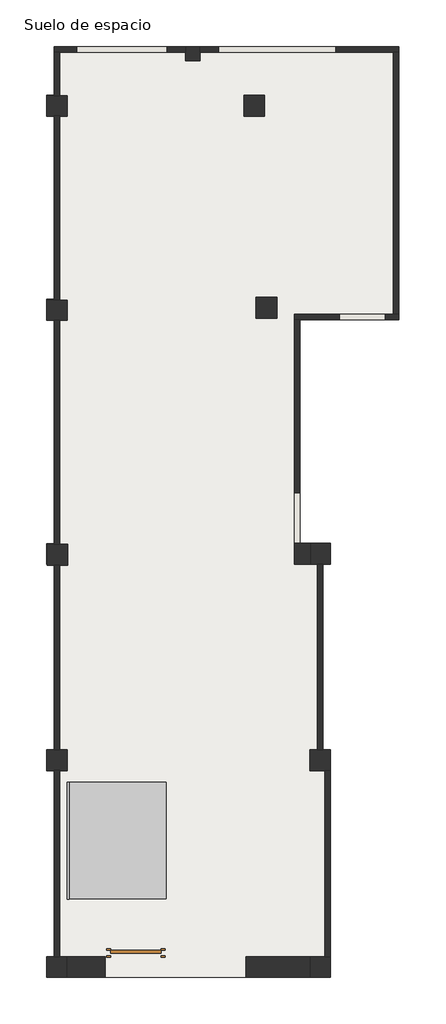
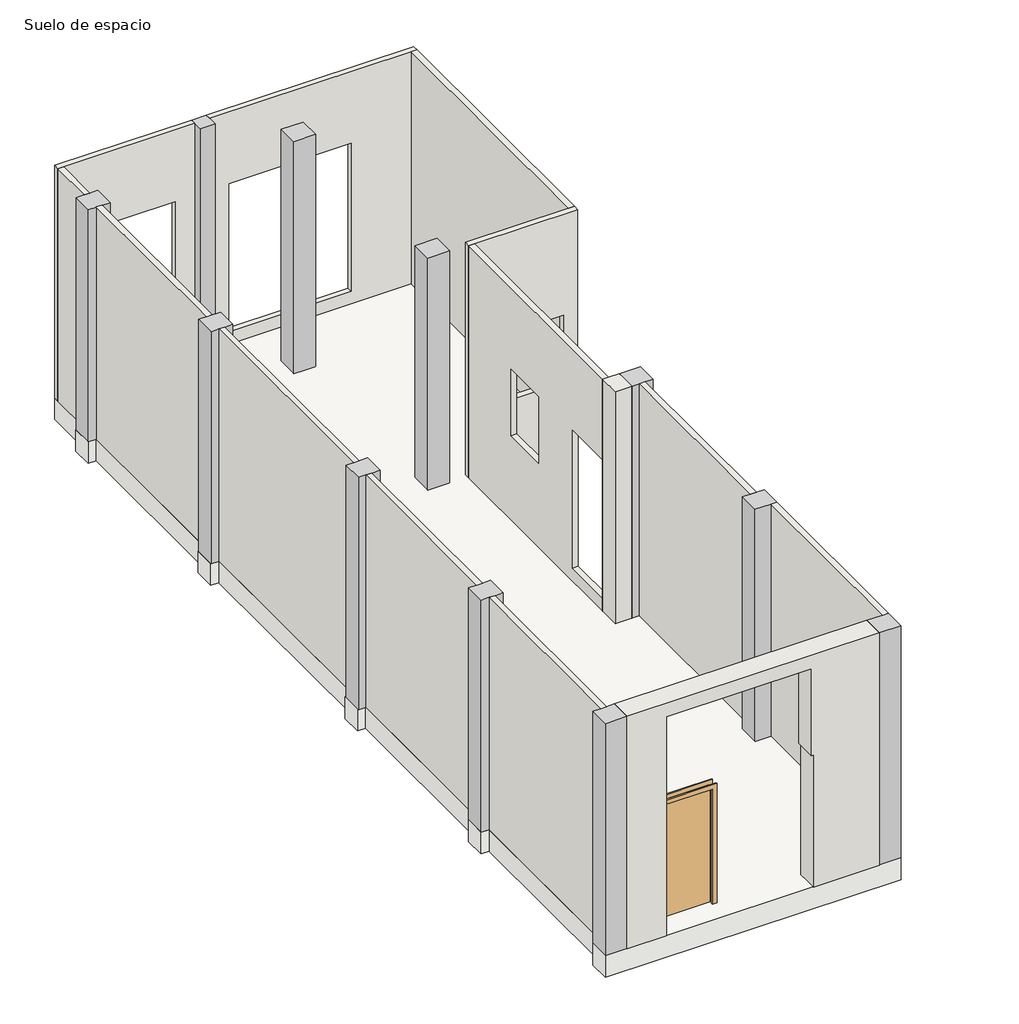
# One storey: 14 walls, 11 columns, 1 door, 1 railing, 1 ramp, 1 slab.
"""IFC4 building model written with IfcOpenShell, lengths in millimetres."""

import ifcopenshell
import ifcopenshell.guid

model = None  # the IFC model being written
_history = None  # IfcOwnerHistory: only IFC2X3 demands one
_inside = {}  # id of a spatial element -> (the spatial element, [elements in it])
_under = {}  # id of a project, library or spatial element -> (it, [spatial elements below it])
_declared = {}  # id of a project -> (the project, [libraries it declares])
_typed = {}  # id of a type object -> (the type object, [elements of that type])
_made_of = {}  # id of a material, layer set ... -> (it, [elements and type objects made of it])


def new_model(schema):
    """Start an empty IFC model of exactly this schema.

    Asked for "IFC4X3", IfcOpenShell would pick the latest addendum, in which some entities
    have other attributes; the version numbers below select the first issue.
    IFC2X3 requires an IfcOwnerHistory on every rooted entity: one is made here for all.
    """
    global model, _history
    if schema == "IFC4X3":
        model = ifcopenshell.file(schema_version=(4, 3, 0, 0))
    else:
        model = ifcopenshell.file(schema=schema)
    _inside.clear()
    _under.clear()
    _declared.clear()
    _typed.clear()
    _made_of.clear()
    _history = None
    if model.schema == "IFC2X3":
        org = make("IfcOrganization", Name="unknown")
        user = make(
            "IfcPersonAndOrganization",
            ThePerson=make("IfcPerson", FamilyName="unknown"),
            TheOrganization=org,
        )
        app = make(
            "IfcApplication",
            ApplicationDeveloper=org,
            Version="unknown",
            ApplicationFullName="unknown",
            ApplicationIdentifier="unknown",
        )
        _history = make(
            "IfcOwnerHistory",
            OwningUser=user,
            OwningApplication=app,
            ChangeAction="ADDED",
            CreationDate=0,
        )
    return model


def make(cls, **values):
    """One entity of the class cls with the attributes given. An attribute that is None is left unset."""
    return model.create_entity(
        cls, **{name: value for name, value in values.items() if value is not None}
    )


def rooted(cls, **values):
    """An entity with a GlobalId (a new one), such as an element, a storey or a relation."""
    return make(cls, GlobalId=ifcopenshell.guid.new(), OwnerHistory=_history, **values)


def si_unit(unit_type, name, prefix=None):
    """IfcSIUnit, for example si_unit("LENGTHUNIT", "METRE", prefix="MILLI")."""
    return make("IfcSIUnit", UnitType=unit_type, Prefix=prefix, Name=name)


def assignment(units):
    """IfcUnitAssignment: the units of a project."""
    return None if units is None else make("IfcUnitAssignment", Units=units)


def point(xyz):
    """IfcCartesianPoint."""
    return None if xyz is None else make("IfcCartesianPoint", Coordinates=xyz)


def direction(xyz):
    """IfcDirection."""
    return None if xyz is None else make("IfcDirection", DirectionRatios=xyz)


def frame(location, z_axis=None, x_axis=None):
    """IfcAxis2Placement3D, a coordinate frame: its origin and axes. An axis left out is left unset."""
    return make(
        "IfcAxis2Placement3D",
        Location=point(location),
        Axis=direction(z_axis),
        RefDirection=direction(x_axis),
    )


def origin():
    """The frame at (0, 0, 0) with its axes left unset."""
    return frame((0.0, 0.0, 0.0))


def origin_with_axes():
    """The frame at (0, 0, 0) with the z axis (0, 0, 1) and the x axis (1, 0, 0) written out."""
    return frame((0.0, 0.0, 0.0), z_axis=(0.0, 0.0, 1.0), x_axis=(1.0, 0.0, 0.0))


def place(relative_to, where):
    """IfcLocalPlacement: puts the frame where relative to a parent placement (None: the world)."""
    return make(
        "IfcLocalPlacement", PlacementRelTo=relative_to, RelativePlacement=where
    )


def context(
    kind, dimensions, precision=None, world=None, true_north=None, identifier=None
):
    """IfcGeometricRepresentationContext, for example the 3D "Model" context."""
    return make(
        "IfcGeometricRepresentationContext",
        ContextIdentifier=identifier,
        ContextType=kind,
        CoordinateSpaceDimension=dimensions,
        Precision=precision,
        WorldCoordinateSystem=world,
        TrueNorth=true_north,
    )


def project(units=None, contexts=None):
    """IfcProject with its units and contexts."""
    return rooted(
        "IfcProject",
        Name="project",
        RepresentationContexts=contexts,
        UnitsInContext=assignment(units),
    )


def spatial(cls, under=None, at=None, **own):
    """A site, building, storey or space (cls), placed at a placement, below another one or the project."""
    s = rooted(cls, ObjectPlacement=at, **own)
    if under is not None:
        _under.setdefault(under.id(), (under, []))[1].append(s)
    return s


def polyline(points):
    """IfcPolyline through the points."""
    return make("IfcPolyline", Points=[point(p) for p in points])


def ellipse_curve(where, semi_axis1, semi_axis2):
    """IfcEllipse in the frame where."""
    return make(
        "IfcEllipse", Position=where, SemiAxis1=semi_axis1, SemiAxis2=semi_axis2
    )


def outline(outer, holes=None, kind="AREA"):
    """IfcArbitraryClosedProfileDef: a profile drawn as a closed curve; with holes, ...WithVoids."""
    if holes is None:
        return make("IfcArbitraryClosedProfileDef", ProfileType=kind, OuterCurve=outer)
    return make(
        "IfcArbitraryProfileDefWithVoids",
        ProfileType=kind,
        OuterCurve=outer,
        InnerCurves=holes,
    )


def extrude(swept, where, along, depth):
    """IfcExtrudedAreaSolid: the profile swept, set in the frame where, extruded along a direction by depth."""
    return make(
        "IfcExtrudedAreaSolid",
        SweptArea=swept,
        Position=where,
        ExtrudedDirection=direction(along),
        Depth=depth,
    )


def faces_of(points, faces, orient=None, outer=None):
    """IfcFace entities. A face is a list of loops; a loop is a list of indices into points, from 0.

    orient and outer hold one flag for each loop. By default every Orientation is true, the
    first loop of a face is its IfcFaceOuterBound and the others are IfcFaceBound.
    """
    made = []
    for i, loops in enumerate(faces):
        bounds = []
        for j, loop in enumerate(loops):
            is_outer = j == 0 if outer is None else outer[i][j]
            bounds.append(
                make(
                    "IfcFaceOuterBound" if is_outer else "IfcFaceBound",
                    Bound=make("IfcPolyLoop", Polygon=[points[k] for k in loop]),
                    Orientation=True if orient is None else orient[i][j],
                )
            )
        made.append(make("IfcFace", Bounds=bounds))
    return made


def faceted_brep(points, faces, orient=None, outer=None, voids=None):
    """IfcFacetedBrep: a solid bounded by flat faces; with voids (closed shells), ...WithVoids."""
    shared = [point(p) for p in points]
    hull = make("IfcClosedShell", CfsFaces=faces_of(shared, faces, orient, outer))
    if voids is None:
        return make("IfcFacetedBrep", Outer=hull)
    return make(
        "IfcFacetedBrepWithVoids",
        Outer=hull,
        Voids=[
            make(cls, CfsFaces=faces_of(shared, fs, o, b)) for cls, fs, o, b in voids
        ],
    )


def shape(context_of_items, identifier, shape_type, items):
    """IfcShapeRepresentation: the items that make up one representation, for example the "Body"."""
    return make(
        "IfcShapeRepresentation",
        ContextOfItems=context_of_items,
        RepresentationIdentifier=identifier,
        RepresentationType=shape_type,
        Items=items,
    )


def source(mapping_origin, context_of_items, identifier, shape_type, items):
    """IfcRepresentationMap: a shape defined once, which mapped items show again and again."""
    return make(
        "IfcRepresentationMap",
        MappingOrigin=mapping_origin,
        MappedRepresentation=shape(context_of_items, identifier, shape_type, items),
    )


def transform(
    local_origin,
    x_axis=None,
    y_axis=None,
    z_axis=None,
    scale=None,
    scale2=None,
    scale3=None,
    uniform=True,
):
    """IfcCartesianTransformationOperator3D, or its non-uniform kind. x_axis, y_axis, z_axis: its Axis1, 2, 3."""
    if uniform:
        return make(
            "IfcCartesianTransformationOperator3D",
            Axis1=direction(x_axis),
            Axis2=direction(y_axis),
            LocalOrigin=point(local_origin),
            Scale=scale,
            Axis3=direction(z_axis),
        )
    return make(
        "IfcCartesianTransformationOperator3DnonUniform",
        Axis1=direction(x_axis),
        Axis2=direction(y_axis),
        LocalOrigin=point(local_origin),
        Scale=scale,
        Axis3=direction(z_axis),
        Scale2=scale2,
        Scale3=scale3,
    )


def mapped(mapping_source, mapping_target):
    """IfcMappedItem: shows the shape of a source again, moved by a transform."""
    return make(
        "IfcMappedItem", MappingSource=mapping_source, MappingTarget=mapping_target
    )


def made_of(thing, what):
    """Note that an element or type object is made of a material, layer set ...; save() writes the relation."""
    if what is not None:
        _made_of.setdefault(what.id(), (what, []))[1].append(thing)
    return thing


def element(
    cls,
    number,
    at=None,
    inside=None,
    cuts=None,
    type_object=None,
    material=None,
    context=None,
    identifier="Body",
    shape_type=None,
    held_by="IfcProductDefinitionShape",
    body=None,
    shapes=None,
    **own,
):
    """One element of the class cls, such as IfcWall. Its Tag is "e" and its number.

    at: its placement. inside: the storey or other place that contains it. cuts: it is an
    opening in that element (IfcRelVoidsElement). A single representation is given by context,
    identifier, shape_type and body (its items); several are given by shapes. held_by: the class
    of the entity that holds the representations. save() writes the other relations.
    """
    e = rooted(cls, Tag="e%d" % number, ObjectPlacement=at, **own)
    if body is not None:
        shapes = [shape(context, identifier, shape_type, body)]
    if shapes is not None:
        e.Representation = make(held_by, Representations=shapes)
    if inside is not None:
        _inside.setdefault(inside.id(), (inside, []))[1].append(e)
    if cuts is not None:
        rooted(
            "IfcRelVoidsElement", RelatingBuildingElement=cuts, RelatedOpeningElement=e
        )
    if type_object is not None:
        _typed.setdefault(type_object.id(), (type_object, []))[1].append(e)
    return made_of(e, material)


def aggregate(whole, parts):
    """IfcRelAggregates: a whole, such as a stair, and the parts it consists of."""
    return rooted("IfcRelAggregates", RelatingObject=whole, RelatedObjects=parts)


def save(model, path):
    """Write the relations noted so far, then the file.

    IfcRelAggregates (storeys below a building ...), IfcRelContainedInSpatialStructure (elements
    in a storey), IfcRelDefinesByType, IfcRelAssociatesMaterial and IfcRelDeclares: one each for
    every whole, place, type object, material and project.
    """
    for whole, parts in _under.values():
        aggregate(whole, parts)
    for where, things in _inside.values():
        rooted(
            "IfcRelContainedInSpatialStructure",
            RelatedElements=things,
            RelatingStructure=where,
        )
    for kind, things in _typed.values():
        rooted("IfcRelDefinesByType", RelatedObjects=things, RelatingType=kind)
    for what, things in _made_of.values():
        rooted("IfcRelAssociatesMaterial", RelatedObjects=things, RelatingMaterial=what)
    for by, libraries in _declared.values():
        rooted("IfcRelDeclares", RelatingContext=by, RelatedDefinitions=libraries)
    model.write(path)


def plane_surface(at):
    """IfcPlane: the flat surface through the origin of the frame at, square to its z axis."""
    return make("IfcPlane", Position=at)


def cylinder_surface(at, radius):
    """IfcCylindricalSurface: all points at the distance radius from the z axis of the frame at."""
    return make("IfcCylindricalSurface", Position=at, Radius=radius)


def advanced_brep(points, edges, surfaces, faces):
    """IfcAdvancedBrep: a solid bounded by faces that lie on surfaces and meet in shared edges.

    An edge is (start, end): straight between two places in points (the first is 0);
    or (start, end, curve); or (start, end, curve, False) where it runs against its curve.
    A face is (place in surfaces, loops), or (place, loops, False) where it looks against
    its surface's normal. A loop lists edges by number (the first is 1), with a minus sign
    where the edge is run from its end to its start. The first loop is the outer one.
    """
    corners = [point(p) for p in points]
    vertices = [make("IfcVertexPoint", VertexGeometry=c) for c in corners]
    made = []
    for start, end, *more in edges:
        made.append(
            make(
                "IfcEdgeCurve",
                EdgeStart=vertices[start],
                EdgeEnd=vertices[end],
                EdgeGeometry=more[0] if more else make("IfcPolyline", Points=[corners[start], corners[end]]),
                SameSense=more[1] if len(more) > 1 else True,
            )
        )
    hull = []
    for where, loops, *sense in faces:
        bounds = []
        for j, loop in enumerate(loops):
            ring = [make("IfcOrientedEdge", EdgeElement=made[abs(k) - 1], Orientation=k > 0) for k in loop]
            bounds.append(
                make(
                    "IfcFaceOuterBound" if j == 0 else "IfcFaceBound",
                    Bound=make("IfcEdgeLoop", EdgeList=ring),
                    Orientation=True,
                )
            )
        hull.append(make("IfcAdvancedFace", Bounds=bounds, FaceSurface=surfaces[where], SameSense=sense[0] if sense else True))
    return make("IfcAdvancedBrep", Outer=make("IfcClosedShell", CfsFaces=hull))


def m_rectangular_column_380_x_380mm_96b74405(model_context):
    return source(origin(), model_context, "Body", "SweptSolid", [
        extrude(outline(polyline([(190.0, 190.0), (190.0, -190.0), (-190.0, -190.0), (-190.0, 190.0), (190.0, 190.0)])), origin_with_axes(), (0.0, 0.0, 1.0), 4300.0),
    ])


def m_single_flush_0915_x_2134mm_17617764(model_context):
    return source(origin(), model_context, "Body", "SweptSolid", [
        extrude(outline(polyline([(2210.0, -533.5), (0.0, -533.5), (0.0, -457.5), (2134.0, -457.5), (2134.0, 457.5), (0.0, 457.5), (0.0, 533.5), (2210.0, 533.5), (2210.0, -533.5)])), frame((0.0, -75.0, 0.0), z_axis=(0.0, 1.0, 0.0), x_axis=(0.0, 0.0, 1.0)), (0.0, 0.0, 1.0), 25.0),
        extrude(outline(polyline([(2210.0, 533.5), (2210.0, -533.5), (0.0, -533.5), (0.0, -457.5), (2134.0, -457.5), (2134.0, 457.5), (0.0, 457.5), (0.0, 533.5), (2210.0, 533.5)])), frame((0.0, 50.0, 0.0), z_axis=(0.0, 1.0, 0.0), x_axis=(0.0, 0.0, 1.0)), (0.0, 0.0, 1.0), 25.0),
        extrude(outline(polyline([(457.5, 1.0), (457.5, -50.0), (-457.5, -50.0), (-457.5, 1.0), (457.5, 1.0)])), origin_with_axes(), (0.0, 0.0, 1.0), 2134.0),
    ])


def ramp_1_1c041b4d(model_context):
    return source(origin(), model_context, "Body", "SweptSolid", [
        extrude(outline(polyline([(-588.7354398, 0.0), (1550.939444, 178.3062403), (1550.939444, 27.7863081), (-588.7354398, -150.5199322), (-588.7354398, 0.0)])), frame((5737.3508412, 0.0, 0.0), z_axis=(1.0, 0.0, 0.0), x_axis=(0.0, 1.0, 0.0)), (0.0, 0.0, 1.0), 1790.0),
    ])


model = new_model("IFC4")

# Units and contexts
model_context = context("Model", 3, world=origin())
ifc_project = project(units=[si_unit("LENGTHUNIT", "METRE", prefix="MILLI")], contexts=[model_context])

# Site, building, storey
site = spatial("IfcSite", under=ifc_project)
building = spatial("IfcBuilding", under=site)
storey = spatial("IfcBuildingStorey", under=building, Name="Suelo de espacio", Elevation=0.0)

# Columns
placement = place(None, origin())
element("IfcColumn", 1, ObjectType="M_Rectangular Column : 260 x 260mm", at=placement, inside=storey, context=model_context, shape_type="Brep", body=[
    faceted_brep([(8142.3508412, 14950.939444, 4300.0), (7882.3508412, 14950.939444, 4300.0), (7882.3508412, 14850.939444, 4300.0), (7882.3508412, 14690.939444, 4300.0), (8142.3508412, 14690.939444, 4300.0), (8142.3508412, 14850.939444, 4300.0), (8142.3508412, 14950.939444, 0.0), (8142.3508412, 14850.939444, 0.0), (8142.3508412, 14690.939444, 0.0), (7882.3508412, 14690.939444, 0.0), (7882.3508412, 14850.939444, 0.0), (7882.3508412, 14950.939444, 0.0)], [[[0, 1, 2, 3, 4, 5]], [[6, 7, 8, 9, 10, 11]], [[1, 0, 6, 11]], [[3, 2, 1, 11, 10, 9]], [[4, 3, 9, 8]], [[0, 5, 4, 8, 7, 6]]]),
])
element("IfcColumn", 2, ObjectType="M_Rectangular Column : 380 x 370mm", at=placement, inside=storey, context=model_context, shape_type="Brep", body=[
    faceted_brep([(5722.3508412, 10330.939444, 4300.0), (5342.3508412, 10330.939444, 4300.0), (5342.3508412, 9960.939444, 4300.0), (5482.3508412, 9960.939444, 4300.0), (5582.3508412, 9960.939444, 4300.0), (5722.3508412, 9960.939444, 4300.0), (5722.3508412, 10330.939444, 0.0), (5722.3508412, 9960.939444, 0.0), (5582.3508412, 9960.939444, 0.0), (5482.3508412, 9960.939444, 0.0), (5342.3508412, 9960.939444, 0.0), (5342.3508412, 10330.939444, 0.0)], [[[0, 1, 2, 3, 4, 5]], [[6, 7, 8, 9, 10, 11]], [[1, 0, 6, 11]], [[2, 1, 11, 10]], [[5, 4, 3, 2, 10, 9, 8, 7]], [[0, 5, 7, 6]]]),
])
element("IfcColumn", 3, ObjectType="M_Rectangular Column : 380 x 370mm", at=placement, inside=storey, context=model_context, shape_type="Brep", body=[
    faceted_brep([(5722.3508412, 14050.939444, 4300.0), (5582.3508412, 14050.939444, 4300.0), (5482.3508412, 14050.939444, 4300.0), (5342.3508412, 14050.939444, 4300.0), (5342.3508412, 13680.939444, 4300.0), (5482.3508412, 13680.939444, 4300.0), (5482.3508412, 13685.939444, 4300.0), (5582.3508412, 13685.939444, 4300.0), (5582.3508412, 13680.939444, 4300.0), (5722.3508412, 13680.939444, 4300.0), (5722.3508412, 14050.939444, 0.0), (5722.3508412, 13680.939444, 0.0), (5582.3508412, 13680.939444, 0.0), (5582.3508412, 13685.939444, 0.0), (5482.3508412, 13685.939444, 0.0), (5482.3508412, 13680.939444, 0.0), (5342.3508412, 13680.939444, 0.0), (5342.3508412, 14050.939444, 0.0), (5482.3508412, 14050.939444, 0.0), (5582.3508412, 14050.939444, 0.0)], [[[0, 1, 2, 3, 4, 5, 6, 7, 8, 9]], [[10, 11, 12, 13, 14, 15, 16, 17, 18, 19]], [[3, 2, 1, 0, 10, 19, 18, 17]], [[4, 3, 17, 16]], [[4, 16, 15, 5]], [[0, 9, 11, 10]], [[7, 13, 12, 8]], [[14, 6, 5, 15]], [[13, 7, 6, 14]], [[11, 9, 8, 12]]]),
])
element("IfcColumn", 4, ObjectType="M_Rectangular Column : 380 x 380mm", at=placement, inside=storey, context=model_context, shape_type="Brep", body=[
    faceted_brep([(5722.3508412, -1629.060556, 4300.0), (5582.3508412, -1629.060556, 4300.0), (5482.3508412, -1629.060556, 4300.0), (5342.3508412, -1629.060556, 4300.0), (5342.3508412, -2009.060556, 4300.0), (5722.3508412, -2009.060556, 4300.0), (5722.3508412, -1629.060556, 0.0), (5722.3508412, -2009.060556, 0.0), (5342.3508412, -2009.060556, 0.0), (5342.3508412, -1629.060556, 0.0), (5482.3508412, -1629.060556, 0.0), (5582.3508412, -1629.060556, 0.0)], [[[0, 1, 2, 3, 4, 5]], [[6, 7, 8, 9, 10, 11]], [[3, 2, 1, 0, 6, 11, 10, 9]], [[4, 3, 9, 8]], [[5, 4, 8, 7]], [[0, 5, 7, 6]]]),
])
element("IfcColumn", 5, ObjectType="M_Rectangular Column : 380 x 380mm", at=placement, inside=storey, context=model_context, shape_type="Brep", body=[
    faceted_brep([(10522.3508412, -1629.060556, 4300.0), (10422.3508412, -1629.060556, 4300.0), (10142.3508412, -1629.060556, 4300.0), (10142.3508412, -2009.060556, 4300.0), (10522.3508412, -2009.060556, 4300.0), (10522.3508412, -1629.060556, 0.0), (10522.3508412, -2009.060556, 0.0), (10142.3508412, -2009.060556, 0.0), (10142.3508412, -1629.060556, 0.0), (10422.3508412, -1629.060556, 0.0)], [[[0, 1, 2, 3, 4]], [[5, 6, 7, 8, 9]], [[2, 1, 0, 5, 9, 8]], [[3, 2, 8, 7]], [[4, 3, 7, 6]], [[0, 4, 6, 5]]]),
])
element("IfcColumn", 6, ObjectType="M_Rectangular Column : 380 x 380mm", at=placement, inside=storey, context=model_context, shape_type="Brep", body=[
    faceted_brep([(5722.3508412, 2140.939444, 4300.0), (5582.3508412, 2140.939444, 4300.0), (5482.3508412, 2140.939444, 4300.0), (5342.3508412, 2140.939444, 4300.0), (5342.3508412, 1760.939444, 4300.0), (5482.3508412, 1760.939444, 4300.0), (5482.3508412, 1761.3849652, 4300.0), (5582.3508412, 1761.3849652, 4300.0), (5582.3508412, 1760.939444, 4300.0), (5722.3508412, 1760.939444, 4300.0), (5722.3508412, 2140.939444, 0.0), (5722.3508412, 1760.939444, 0.0), (5582.3508412, 1760.939444, 0.0), (5582.3508412, 1761.3849652, 0.0), (5482.3508412, 1761.3849652, 0.0), (5482.3508412, 1760.939444, 0.0), (5342.3508412, 1760.939444, 0.0), (5342.3508412, 2140.939444, 0.0), (5482.3508412, 2140.939444, 0.0), (5582.3508412, 2140.939444, 0.0)], [[[0, 1, 2, 3, 4, 5, 6, 7, 8, 9]], [[10, 11, 12, 13, 14, 15, 16, 17, 18, 19]], [[3, 2, 1, 0, 10, 19, 18, 17]], [[4, 3, 17, 16]], [[4, 16, 15, 5]], [[0, 9, 11, 10]], [[7, 13, 12, 8]], [[14, 6, 5, 15]], [[11, 9, 8, 12]], [[13, 7, 6, 14]]]),
])
element("IfcColumn", 7, ObjectType="M_Rectangular Column : 380 x 380mm", at=placement, inside=storey, context=model_context, shape_type="Brep", body=[
    faceted_brep([(10522.3508412, 2140.939444, 4300.0), (10382.3508412, 2140.939444, 4300.0), (10282.3508412, 2140.939444, 4300.0), (10142.3508412, 2140.939444, 4300.0), (10142.3508412, 1760.939444, 4300.0), (10422.3508412, 1760.939444, 4300.0), (10522.3508412, 1760.939444, 4300.0), (10522.3508412, 2140.939444, 0.0), (10522.3508412, 1760.939444, 0.0), (10422.3508412, 1760.939444, 0.0), (10142.3508412, 1760.939444, 0.0), (10142.3508412, 2140.939444, 0.0), (10282.3508412, 2140.939444, 0.0), (10382.3508412, 2140.939444, 0.0)], [[[0, 1, 2, 3, 4, 5, 6]], [[7, 8, 9, 10, 11, 12, 13]], [[3, 2, 1, 0, 7, 13, 12, 11]], [[4, 3, 11, 10]], [[6, 5, 4, 10, 9, 8]], [[0, 6, 8, 7]]]),
])
element("IfcColumn", 8, ObjectType="M_Rectangular Column : 380 x 380mm", at=placement, inside=storey, context=model_context, shape_type="Brep", body=[
    faceted_brep([(5732.3508412, 5880.939444, 4300.0), (5582.3508412, 5880.939444, 4300.0), (5482.3508412, 5880.939444, 4300.0), (5352.3508412, 5880.939444, 4300.0), (5352.3508412, 5500.939444, 4300.0), (5482.3508412, 5500.939444, 4300.0), (5582.3508412, 5500.939444, 4300.0), (5732.3508412, 5500.939444, 4300.0), (5732.3508412, 5880.939444, 0.0), (5732.3508412, 5500.939444, 0.0), (5582.3508412, 5500.939444, 0.0), (5482.3508412, 5500.939444, 0.0), (5352.3508412, 5500.939444, 0.0), (5352.3508412, 5880.939444, 0.0), (5482.3508412, 5880.939444, 0.0), (5582.3508412, 5880.939444, 0.0)], [[[0, 1, 2, 3, 4, 5, 6, 7]], [[8, 9, 10, 11, 12, 13, 14, 15]], [[3, 2, 1, 0, 8, 15, 14, 13]], [[4, 3, 13, 12]], [[7, 6, 5, 4, 12, 11, 10, 9]], [[0, 7, 9, 8]]]),
])
element("IfcColumn", 9, ObjectType="M_Rectangular Column : 380 x 380mm", at=placement, inside=storey, context=model_context, shape_type="Brep", body=[
    faceted_brep([(10522.3508412, 5520.939444, 4300.0), (10522.3508412, 5900.939444, 4300.0), (10152.3508412, 5900.939444, 4300.0), (10152.3508412, 5520.939444, 4300.0), (10282.3508412, 5520.939444, 4300.0), (10382.3508412, 5520.939444, 4300.0), (10522.3508412, 5900.939444, 0.0), (10522.3508412, 5520.939444, 0.0), (10382.3508412, 5520.939444, 0.0), (10282.3508412, 5520.939444, 0.0), (10152.3508412, 5520.939444, 0.0), (10152.3508412, 5900.939444, 0.0)], [[[0, 1, 2, 3, 4, 5]], [[6, 7, 8, 9, 10, 11]], [[1, 6, 11, 2]], [[7, 0, 5, 4, 3, 10, 9, 8]], [[1, 0, 7, 6]], [[3, 2, 11, 10]]]),
])
m_rectangular_column_380_x_380mm_shape = m_rectangular_column_380_x_380mm_96b74405(model_context)
element("IfcColumn", 10, ObjectType="M_Rectangular Column : 380 x 380mm", at=placement, inside=storey, context=model_context, shape_type="MappedRepresentation", body=[
    mapped(m_rectangular_column_380_x_380mm_shape, transform((9132.3508412, 13870.939444, 0.0), x_axis=(1.0, 0.0, 0.0), y_axis=(0.0, 1.0, 0.0), z_axis=(0.0, 0.0, 1.0))),
])
element("IfcColumn", 11, ObjectType="M_Rectangular Column : 380 x 380mm", at=placement, inside=storey, context=model_context, shape_type="MappedRepresentation", body=[
    mapped(m_rectangular_column_380_x_380mm_shape, transform((9352.3508412, 10190.939444, 0.0), x_axis=(1.0, 0.0, 0.0), y_axis=(0.0, 1.0, 0.0), z_axis=(0.0, 0.0, 1.0))),
])

# Door
m_single_flush_0915_x_2134mm_shape = m_single_flush_0915_x_2134mm_17617764(model_context)
element("IfcDoor", 12, ObjectType="M_Single-Flush : 0915 x 2134mm", at=placement, inside=storey, context=model_context, shape_type="MappedRepresentation", body=[
    mapped(m_single_flush_0915_x_2134mm_shape, transform((6972.3508412, -1564.060556, 0.0), x_axis=(-1.0, 0.0, 0.0), y_axis=(0.0, -1.0, 0.0), z_axis=(0.0, 0.0, 1.0))),
])

# Railing
element("IfcRailing", 13, ObjectType="900mm Pipe", at=placement, inside=storey, context=model_context, shape_type="AdvancedBrep", body=[
    advanced_brep(
    [(5757.3508412, -588.7354398, 879.9306757), (5717.3508412, -588.7354398, 879.9306757), (5757.3508412, 1550.939444, 1058.236916), (5717.3508412, 1550.939444, 1058.236916)],
    [
        (0, 1, ellipse_curve(frame((5737.3508412, -588.7354398, 879.9306757), z_axis=(0.0, -1.0, 0.0), x_axis=(0.0, 0.0, -0.9999999999999999)), 20.0693243, 20.0)),
        (1, 0, ellipse_curve(frame((5737.3508412, -588.7354398, 879.9306757), z_axis=(0.0, -1.0, 0.0), x_axis=(0.0, 0.0, -0.9999999999999999)), 20.0693243, 20.0)),
        (2, 3, ellipse_curve(frame((5737.3508412, 1550.939444, 1058.236916), z_axis=(0.0, 1.0, 0.0), x_axis=(0.0, 0.0, -0.9999999999999999)), 20.0693243, 20.0)),
        (3, 2, ellipse_curve(frame((5737.3508412, 1550.939444, 1058.236916), z_axis=(0.0, 1.0, 0.0), x_axis=(0.0, 0.0, -0.9999999999999999)), 20.0693243, 20.0)),
        (0, 2),
        (3, 1),
    ],
    [
        plane_surface(frame((5737.3508412, -588.7354398, 900.0), z_axis=(0.0, -1.0, 0.0), x_axis=(0.0, 0.0, 1.0))),
        plane_surface(frame((5737.3508412, 1550.939444, 1078.3062403), z_axis=(0.0, 1.0, 0.0), x_axis=(0.0, 0.0, 1.0))),
        cylinder_surface(frame((5737.3508412, -587.0745302, 880.0690848), z_axis=(0.0, -0.9965457582448797, -0.08304547985373997), x_axis=(-1.0, 0.0, 0.0)), 20.0),
    ],
    [
        (0, [[1, 2]]),
        (1, [[3, 4]]),
        (2, [[-1, 5, -4, 6]]),
        (2, [[-2, -6, -3, -5]]),
    ],
),
    advanced_brep(
    [(5722.3508412, -588.7354398, 759.9480068), (5752.3508412, -588.7354398, 759.9480068), (5722.3508412, 1550.939444, 938.2542471), (5752.3508412, 1550.939444, 938.2542471)],
    [
        (0, 1, ellipse_curve(frame((5737.3508412, -588.7354398, 759.9480068), z_axis=(0.0, -1.0, 0.0), x_axis=(0.0, 0.0, -1.0)), 15.0519932, 15.0)),
        (1, 0, ellipse_curve(frame((5737.3508412, -588.7354398, 759.9480068), z_axis=(0.0, -1.0, 0.0), x_axis=(0.0, 0.0, -1.0)), 15.0519932, 15.0)),
        (2, 3, ellipse_curve(frame((5737.3508412, 1550.939444, 938.2542471), z_axis=(0.0, 1.0, 0.0), x_axis=(0.0, 0.0, -1.0)), 15.0519932, 15.0)),
        (3, 2, ellipse_curve(frame((5737.3508412, 1550.939444, 938.2542471), z_axis=(0.0, 1.0, 0.0), x_axis=(0.0, 0.0, -1.0)), 15.0519932, 15.0)),
        (0, 2),
        (3, 1),
    ],
    [
        plane_surface(frame((5737.3508412, -588.7354398, 775.0), z_axis=(0.0, -1.0, 0.0), x_axis=(0.0, 0.0, 1.0))),
        plane_surface(frame((5737.3508412, 1550.939444, 953.3062403), z_axis=(0.0, 1.0, 0.0), x_axis=(0.0, 0.0, 1.0))),
        cylinder_surface(frame((5737.3508412, -587.4897576, 760.0518136), z_axis=(0.0, -0.9965457582448797, -0.08304547985373999), x_axis=(1.0, 0.0, 0.0)), 15.0),
    ],
    [
        (0, [[1, 2]]),
        (1, [[3, 4]]),
        (2, [[-1, 5, -4, 6]]),
        (2, [[-2, -6, -3, -5]]),
    ],
),
    advanced_brep(
    [(5722.3508412, -588.7354398, 634.9480068), (5752.3508412, -588.7354398, 634.9480068), (5722.3508412, 1550.939444, 813.2542471), (5752.3508412, 1550.939444, 813.2542471)],
    [
        (0, 1, ellipse_curve(frame((5737.3508412, -588.7354398, 634.9480068), z_axis=(0.0, -1.0, 0.0), x_axis=(0.0, 0.0, -1.0)), 15.0519932, 15.0)),
        (1, 0, ellipse_curve(frame((5737.3508412, -588.7354398, 634.9480068), z_axis=(0.0, -1.0, 0.0), x_axis=(0.0, 0.0, -1.0)), 15.0519932, 15.0)),
        (2, 3, ellipse_curve(frame((5737.3508412, 1550.939444, 813.2542471), z_axis=(0.0, 1.0, 0.0), x_axis=(0.0, 0.0, -1.0)), 15.0519932, 15.0)),
        (3, 2, ellipse_curve(frame((5737.3508412, 1550.939444, 813.2542471), z_axis=(0.0, 1.0, 0.0), x_axis=(0.0, 0.0, -1.0)), 15.0519932, 15.0)),
        (0, 2),
        (3, 1),
    ],
    [
        plane_surface(frame((5737.3508412, -588.7354398, 650.0), z_axis=(0.0, -1.0, 0.0), x_axis=(0.0, 0.0, 1.0))),
        plane_surface(frame((5737.3508412, 1550.939444, 828.3062403), z_axis=(0.0, 1.0, 0.0), x_axis=(0.0, 0.0, 1.0))),
        cylinder_surface(frame((5737.3508412, -587.4897576, 635.0518136), z_axis=(0.0, -0.9965457582448797, -0.08304547985373999), x_axis=(1.0, 0.0, 0.0)), 15.0),
    ],
    [
        (0, [[1, 2]]),
        (1, [[3, 4]]),
        (2, [[-1, 5, -4, 6]]),
        (2, [[-2, -6, -3, -5]]),
    ],
),
    advanced_brep(
    [(5722.3508412, -588.7354398, 509.9480068), (5752.3508412, -588.7354398, 509.9480068), (5722.3508412, 1550.939444, 688.2542471), (5752.3508412, 1550.939444, 688.2542471)],
    [
        (0, 1, ellipse_curve(frame((5737.3508412, -588.7354398, 509.9480068), z_axis=(0.0, -1.0, 0.0), x_axis=(0.0, 0.0, -1.0)), 15.0519932, 15.0)),
        (1, 0, ellipse_curve(frame((5737.3508412, -588.7354398, 509.9480068), z_axis=(0.0, -1.0, 0.0), x_axis=(0.0, 0.0, -1.0)), 15.0519932, 15.0)),
        (2, 3, ellipse_curve(frame((5737.3508412, 1550.939444, 688.2542471), z_axis=(0.0, 1.0, 0.0), x_axis=(0.0, 0.0, -1.0)), 15.0519932, 15.0)),
        (3, 2, ellipse_curve(frame((5737.3508412, 1550.939444, 688.2542471), z_axis=(0.0, 1.0, 0.0), x_axis=(0.0, 0.0, -1.0)), 15.0519932, 15.0)),
        (0, 2),
        (3, 1),
    ],
    [
        plane_surface(frame((5737.3508412, -588.7354398, 525.0), z_axis=(0.0, -1.0, 0.0), x_axis=(0.0, 0.0, 1.0))),
        plane_surface(frame((5737.3508412, 1550.939444, 703.3062403), z_axis=(0.0, 1.0, 0.0), x_axis=(0.0, 0.0, 1.0))),
        cylinder_surface(frame((5737.3508412, -587.4897576, 510.0518136), z_axis=(0.0, -0.9965457582448797, -0.08304547985373999), x_axis=(1.0, 0.0, 0.0)), 15.0),
    ],
    [
        (0, [[1, 2]]),
        (1, [[3, 4]]),
        (2, [[-1, 5, -4, 6]]),
        (2, [[-2, -6, -3, -5]]),
    ],
),
    advanced_brep(
    [(5722.3508412, -588.7354398, 384.9480068), (5752.3508412, -588.7354398, 384.9480068), (5722.3508412, 1550.939444, 563.2542471), (5752.3508412, 1550.939444, 563.2542471)],
    [
        (0, 1, ellipse_curve(frame((5737.3508412, -588.7354398, 384.9480068), z_axis=(0.0, -1.0, 0.0), x_axis=(0.0, 0.0, -1.0)), 15.0519932, 15.0)),
        (1, 0, ellipse_curve(frame((5737.3508412, -588.7354398, 384.9480068), z_axis=(0.0, -1.0, 0.0), x_axis=(0.0, 0.0, -1.0)), 15.0519932, 15.0)),
        (2, 3, ellipse_curve(frame((5737.3508412, 1550.939444, 563.2542471), z_axis=(0.0, 1.0, 0.0), x_axis=(0.0, 0.0, -1.0)), 15.0519932, 15.0)),
        (3, 2, ellipse_curve(frame((5737.3508412, 1550.939444, 563.2542471), z_axis=(0.0, 1.0, 0.0), x_axis=(0.0, 0.0, -1.0)), 15.0519932, 15.0)),
        (0, 2),
        (3, 1),
    ],
    [
        plane_surface(frame((5737.3508412, -588.7354398, 400.0), z_axis=(0.0, -1.0, 0.0), x_axis=(0.0, 0.0, 1.0))),
        plane_surface(frame((5737.3508412, 1550.939444, 578.3062403), z_axis=(0.0, 1.0, 0.0), x_axis=(0.0, 0.0, 1.0))),
        cylinder_surface(frame((5737.3508412, -587.4897576, 385.0518136), z_axis=(0.0, -0.9965457582448797, -0.08304547985373996), x_axis=(1.0, 0.0, 0.0)), 15.0),
    ],
    [
        (0, [[1, 2]]),
        (1, [[3, 4]]),
        (2, [[-1, 5, -4, 6]]),
        (2, [[-2, -6, -3, -5]]),
    ],
),
    advanced_brep(
    [(5722.3508412, -588.7354398, 259.9480068), (5752.3508412, -588.7354398, 259.9480068), (5722.3508412, 1550.939444, 438.2542471), (5752.3508412, 1550.939444, 438.2542471)],
    [
        (0, 1, ellipse_curve(frame((5737.3508412, -588.7354398, 259.9480068), z_axis=(0.0, -1.0, 0.0), x_axis=(0.0, 0.0, -1.0)), 15.0519932, 15.0)),
        (1, 0, ellipse_curve(frame((5737.3508412, -588.7354398, 259.9480068), z_axis=(0.0, -1.0, 0.0), x_axis=(0.0, 0.0, -1.0)), 15.0519932, 15.0)),
        (2, 3, ellipse_curve(frame((5737.3508412, 1550.939444, 438.2542471), z_axis=(0.0, 1.0, 0.0), x_axis=(0.0, 0.0, -1.0)), 15.0519932, 15.0)),
        (3, 2, ellipse_curve(frame((5737.3508412, 1550.939444, 438.2542471), z_axis=(0.0, 1.0, 0.0), x_axis=(0.0, 0.0, -1.0)), 15.0519932, 15.0)),
        (0, 2),
        (3, 1),
    ],
    [
        plane_surface(frame((5737.3508412, -588.7354398, 275.0), z_axis=(0.0, -1.0, 0.0), x_axis=(0.0, 0.0, 1.0))),
        plane_surface(frame((5737.3508412, 1550.939444, 453.3062403), z_axis=(0.0, 1.0, 0.0), x_axis=(0.0, 0.0, 1.0))),
        cylinder_surface(frame((5737.3508412, -587.4897576, 260.0518136), z_axis=(0.0, -0.9965457582448797, -0.08304547985373996), x_axis=(1.0, 0.0, 0.0)), 15.0),
    ],
    [
        (0, [[1, 2]]),
        (1, [[3, 4]]),
        (2, [[-1, 5, -4, 6]]),
        (2, [[-2, -6, -3, -5]]),
    ],
),
    advanced_brep(
    [(5722.3508412, -588.7354398, 134.9480068), (5752.3508412, -588.7354398, 134.9480068), (5722.3508412, 1550.939444, 313.2542471), (5752.3508412, 1550.939444, 313.2542471)],
    [
        (0, 1, ellipse_curve(frame((5737.3508412, -588.7354398, 134.9480068), z_axis=(0.0, -1.0, 0.0), x_axis=(0.0, 0.0, -1.0)), 15.0519932, 15.0)),
        (1, 0, ellipse_curve(frame((5737.3508412, -588.7354398, 134.9480068), z_axis=(0.0, -1.0, 0.0), x_axis=(0.0, 0.0, -1.0)), 15.0519932, 15.0)),
        (2, 3, ellipse_curve(frame((5737.3508412, 1550.939444, 313.2542471), z_axis=(0.0, 1.0, 0.0), x_axis=(0.0, 0.0, -1.0)), 15.0519932, 15.0)),
        (3, 2, ellipse_curve(frame((5737.3508412, 1550.939444, 313.2542471), z_axis=(0.0, 1.0, 0.0), x_axis=(0.0, 0.0, -1.0)), 15.0519932, 15.0)),
        (0, 2),
        (3, 1),
    ],
    [
        plane_surface(frame((5737.3508412, -588.7354398, 150.0), z_axis=(0.0, -1.0, 0.0), x_axis=(0.0, 0.0, 1.0))),
        plane_surface(frame((5737.3508412, 1550.939444, 328.3062403), z_axis=(0.0, 1.0, 0.0), x_axis=(0.0, 0.0, 1.0))),
        cylinder_surface(frame((5737.3508412, -587.4897576, 135.0518136), z_axis=(0.0, -0.9965457582448797, -0.08304547985373996), x_axis=(1.0, 0.0, 0.0)), 15.0),
    ],
    [
        (0, [[1, 2]]),
        (1, [[3, 4]]),
        (2, [[-1, 5, -4, 6]]),
        (2, [[-2, -6, -3, -5]]),
    ],
),
    advanced_brep(
    [(5749.8508412, 1411.2645602, 1026.5280181), (5749.8508412, 1411.2645602, 166.6666667), (5724.8508412, 1411.2645602, 166.6666667), (5724.8508412, 1411.2645602, 1026.5280181)],
    [
        (0, 1),
        (1, 2, ellipse_curve(frame((5737.3508412, 1411.2645602, 166.6666667), z_axis=(0.0, -0.08304547985373995, 0.9965457582448797), x_axis=(0.0, 0.9965457582448798, 0.08304547985373882)), 12.5433277, 12.5)),
        (2, 3),
        (3, 0, ellipse_curve(frame((5737.3508412, 1411.2645602, 1026.5280181), z_axis=(0.0, 0.08304547985373997, -0.9965457582448797), x_axis=(0.0, 0.9965457582448797, 0.0830454798537388)), 12.5433277, 12.5)),
        (0, 3, ellipse_curve(frame((5737.3508412, 1411.2645602, 1026.5280181), z_axis=(0.0, 0.08304547985373997, -0.9965457582448797), x_axis=(0.0, 0.9965457582448797, 0.0830454798537388)), 12.5433277, 12.5)),
        (2, 1, ellipse_curve(frame((5737.3508412, 1411.2645602, 166.6666667), z_axis=(0.0, -0.08304547985373995, 0.9965457582448797), x_axis=(0.0, 0.9965457582448798, 0.08304547985373882)), 12.5433277, 12.5)),
    ],
    [
        cylinder_surface(frame((5737.3508412, 1411.2645602, 66.6666667), z_axis=(0.0, 0.0, 1.0), x_axis=(-1.0, 0.0, 0.0)), 12.5),
        plane_surface(frame((5712.3508412, 1436.2645602, 1028.6113514), z_axis=(0.0, -0.08304547985373997, 0.9965457582448797), x_axis=(1.0, 0.0, 0.0))),
        plane_surface(frame((5712.3508412, 1386.2645602, 164.5833333), z_axis=(0.0, 0.08304547985373995, -0.9965457582448797), x_axis=(1.0, 0.0, 0.0))),
    ],
    [
        (0, [[1, 2, 3, 4]]),
        (0, [[-1, 5, -3, 6]]),
        (1, [[-4, -5]]),
        (2, [[-2, -6]]),
    ],
),
    advanced_brep(
    [(5749.8508412, 411.2645602, 943.1946847), (5749.8508412, 411.2645602, 83.3333333), (5724.8508412, 411.2645602, 83.3333333), (5724.8508412, 411.2645602, 943.1946847)],
    [
        (0, 1),
        (1, 2, ellipse_curve(frame((5737.3508412, 411.2645602, 83.3333333), z_axis=(0.0, -0.08304547985373995, 0.9965457582448797), x_axis=(0.0, 0.9965457582448798, 0.08304547985373882)), 12.5433277, 12.5)),
        (2, 3),
        (3, 0, ellipse_curve(frame((5737.3508412, 411.2645602, 943.1946847), z_axis=(0.0, 0.08304547985373997, -0.9965457582448797), x_axis=(0.0, 0.9965457582448797, 0.0830454798537388)), 12.5433277, 12.5)),
        (0, 3, ellipse_curve(frame((5737.3508412, 411.2645602, 943.1946847), z_axis=(0.0, 0.08304547985373997, -0.9965457582448797), x_axis=(0.0, 0.9965457582448797, 0.0830454798537388)), 12.5433277, 12.5)),
        (2, 1, ellipse_curve(frame((5737.3508412, 411.2645602, 83.3333333), z_axis=(0.0, -0.08304547985373995, 0.9965457582448797), x_axis=(0.0, 0.9965457582448798, 0.08304547985373882)), 12.5433277, 12.5)),
    ],
    [
        cylinder_surface(frame((5737.3508412, 411.2645602, -16.6666667), z_axis=(0.0, 0.0, 1.0), x_axis=(-1.0, 0.0, 0.0)), 12.5),
        plane_surface(frame((5712.3508412, 436.2645602, 945.2780181), z_axis=(0.0, -0.08304547985373997, 0.9965457582448797), x_axis=(1.0, 0.0, 0.0))),
        plane_surface(frame((5712.3508412, 386.2645602, 81.25), z_axis=(0.0, 0.08304547985373995, -0.9965457582448797), x_axis=(1.0, 0.0, 0.0))),
    ],
    [
        (0, [[1, 2, 3, 4]]),
        (0, [[-1, 5, -3, 6]]),
        (1, [[-4, -5]]),
        (2, [[-2, -6]]),
    ],
),
    advanced_brep(
    [(5749.8508412, 1538.439444, 1037.1259251), (5749.8508412, 1538.439444, 177.2645736), (5724.8508412, 1538.439444, 177.2645736), (5724.8508412, 1538.439444, 1037.1259251)],
    [
        (0, 1),
        (1, 2, ellipse_curve(frame((5737.3508412, 1538.439444, 177.2645736), z_axis=(0.0, -0.08304547985373995, 0.9965457582448797), x_axis=(0.0, 0.9965457582448798, 0.08304547985373882)), 12.5433277, 12.5)),
        (2, 3),
        (3, 0, ellipse_curve(frame((5737.3508412, 1538.439444, 1037.1259251), z_axis=(0.0, 0.08304547985373997, -0.9965457582448797), x_axis=(0.0, 0.9965457582448797, 0.0830454798537388)), 12.5433277, 12.5)),
        (0, 3, ellipse_curve(frame((5737.3508412, 1538.439444, 1037.1259251), z_axis=(0.0, 0.08304547985373997, -0.9965457582448797), x_axis=(0.0, 0.9965457582448797, 0.0830454798537388)), 12.5433277, 12.5)),
        (2, 1, ellipse_curve(frame((5737.3508412, 1538.439444, 177.2645736), z_axis=(0.0, -0.08304547985373995, 0.9965457582448797), x_axis=(0.0, 0.9965457582448798, 0.08304547985373882)), 12.5433277, 12.5)),
    ],
    [
        cylinder_surface(frame((5737.3508412, 1538.439444, 77.2645736), z_axis=(0.0, 0.0, 1.0), x_axis=(-1.0, 0.0, 0.0)), 12.5),
        plane_surface(frame((5712.3508412, 1563.439444, 1039.2092584), z_axis=(0.0, -0.08304547985373997, 0.9965457582448797), x_axis=(1.0, 0.0, 0.0))),
        plane_surface(frame((5712.3508412, 1513.439444, 175.1812403), z_axis=(0.0, 0.08304547985373995, -0.9965457582448797), x_axis=(1.0, 0.0, 0.0))),
    ],
    [
        (0, [[1, 2, 3, 4]]),
        (0, [[-1, 5, -3, 6]]),
        (1, [[-4, -5]]),
        (2, [[-2, -6]]),
    ],
),
    advanced_brep(
    [(5749.8508412, -576.2354398, 860.9030181), (5749.8508412, -576.2354398, 1.0416667), (5724.8508412, -576.2354398, 1.0416667), (5724.8508412, -576.2354398, 860.9030181)],
    [
        (0, 1),
        (1, 2, ellipse_curve(frame((5737.3508412, -576.2354398, 1.0416667), z_axis=(0.0, -0.08304547985373995, 0.9965457582448797), x_axis=(0.0, 0.9965457582448798, 0.08304547985373882)), 12.5433277, 12.5)),
        (2, 3),
        (3, 0, ellipse_curve(frame((5737.3508412, -576.2354398, 860.9030181), z_axis=(0.0, 0.08304547985373997, -0.9965457582448797), x_axis=(0.0, 0.9965457582448797, 0.0830454798537388)), 12.5433277, 12.5)),
        (0, 3, ellipse_curve(frame((5737.3508412, -576.2354398, 860.9030181), z_axis=(0.0, 0.08304547985373997, -0.9965457582448797), x_axis=(0.0, 0.9965457582448797, 0.0830454798537388)), 12.5433277, 12.5)),
        (2, 1, ellipse_curve(frame((5737.3508412, -576.2354398, 1.0416667), z_axis=(0.0, -0.08304547985373995, 0.9965457582448797), x_axis=(0.0, 0.9965457582448798, 0.08304547985373882)), 12.5433277, 12.5)),
    ],
    [
        cylinder_surface(frame((5737.3508412, -576.2354398, -98.9583333), z_axis=(0.0, 0.0, 1.0), x_axis=(-1.0, 0.0, 0.0)), 12.5),
        plane_surface(frame((5712.3508412, -551.2354398, 862.9863514), z_axis=(0.0, -0.08304547985373997, 0.9965457582448797), x_axis=(1.0, 0.0, 0.0))),
        plane_surface(frame((5712.3508412, -601.2354398, -1.0416667), z_axis=(0.0, 0.08304547985373995, -0.9965457582448797), x_axis=(1.0, 0.0, 0.0))),
    ],
    [
        (0, [[1, 2, 3, 4]]),
        (0, [[-1, 5, -3, 6]]),
        (1, [[-4, -5]]),
        (2, [[-2, -6]]),
    ],
),
])

# Ramp
ramp_1_shape = ramp_1_1c041b4d(model_context)
element("IfcRamp", 14, ObjectType="Ramp 1", at=placement, inside=storey, context=model_context, shape_type="MappedRepresentation", body=[
    mapped(ramp_1_shape, transform((0.0, 0.0, 0.0), x_axis=(1.0, 0.0, 0.0), y_axis=(0.0, 1.0, 0.0), z_axis=(0.0, 0.0, 1.0))),
])

# Slab
element("IfcSlab", 15, ObjectType="Generic Floor - 400mm", at=placement, inside=storey, context=model_context, shape_type="SweptSolid", body=[
    extrude(outline(polyline([(11772.3508412, 14950.939444), (11772.3508412, 9970.939444), (9962.3508412, 9970.939444), (9962.3508412, 5900.939444), (10382.3508412, 5900.939444), (10382.3508412, 2140.939444), (10522.3508412, 2140.939444), (10522.3508412, -2009.060556), (5342.3508412, -2009.060556), (5342.3508412, -1629.060556), (5482.3508412, -1629.060556), (5482.3508412, 1761.3849652), (5342.3508412, 1761.3849652), (5342.3508412, 2140.939444), (5482.3508412, 2140.939444), (5482.3508412, 5516.6200626), (5342.3508412, 5516.6200626), (5342.3508412, 5896.6200626), (5482.3508412, 5896.6200626), (5482.3508412, 9965.939444), (5342.3508412, 9965.939444), (5342.3508412, 10345.939444), (5482.3508412, 10345.939444), (5482.3508412, 13690.939444), (5342.3508412, 13690.939444), (5342.3508412, 14060.939444), (5482.3508412, 14060.939444), (5482.3508412, 14950.939444), (11772.3508412, 14950.939444)])), frame((0.0, 0.0, -400.0), z_axis=(0.0, 0.0, 1.0), x_axis=(1.0, 0.0, 0.0)), (0.0, 0.0, 1.0), 400.0),
])

# Walls
element("IfcWall", 16, ObjectType="Generic - 100mm Masonry", at=placement, inside=storey, context=model_context, shape_type="Brep", body=[
    faceted_brep([(5582.3508412, -1629.060556, 0.0), (5582.3508412, 1760.939444, 0.0), (5582.3508412, 1761.3849652, 0.0), (5582.3508412, 1761.3849652, 4300.0), (5582.3508412, 1760.939444, 4300.0), (5582.3508412, -1629.060556, 4300.0), (5482.3508412, -1629.060556, 0.0), (5482.3508412, -1629.060556, 4300.0), (5482.3508412, 1760.939444, 4300.0), (5482.3508412, 1761.3849652, 4300.0), (5482.3508412, 1761.3849652, 0.0), (5482.3508412, 1760.939444, 0.0)], [[[0, 1, 2, 3, 4, 5]], [[6, 7, 8, 9, 10, 11]], [[2, 1, 0, 6, 11, 10]], [[3, 2, 10, 9]], [[5, 4, 3, 9, 8, 7]], [[0, 5, 7, 6]]]),
])
element("IfcWall", 17, ObjectType="Generic - 100mm Masonry", at=placement, inside=storey, context=model_context, shape_type="SweptSolid", body=[
    extrude(outline(polyline([(5582.3508412, 5500.939444), (5582.3508412, 2140.939444), (5482.3508412, 2140.939444), (5482.3508412, 5500.939444), (5582.3508412, 5500.939444)])), origin_with_axes(), (0.0, 0.0, 1.0), 4300.0),
])
element("IfcWall", 18, ObjectType="Generic - 100mm Masonry", at=placement, inside=storey, context=model_context, shape_type="SweptSolid", body=[
    extrude(outline(polyline([(5582.3508412, 9960.939444), (5582.3508412, 5880.939444), (5482.3508412, 5880.939444), (5482.3508412, 9960.939444), (5582.3508412, 9960.939444)])), origin_with_axes(), (0.0, 0.0, 1.0), 4300.0),
])
element("IfcWall", 19, ObjectType="Generic - 100mm Masonry", at=placement, inside=storey, context=model_context, shape_type="Brep", body=[
    faceted_brep([(5582.3508412, 10335.939444, 0.0), (5582.3508412, 13680.939444, 0.0), (5582.3508412, 13685.939444, 0.0), (5582.3508412, 13685.939444, 4300.0), (5582.3508412, 13680.939444, 4300.0), (5582.3508412, 10335.939444, 4300.0), (5482.3508412, 10335.939444, 0.0), (5482.3508412, 10335.939444, 4300.0), (5482.3508412, 13680.939444, 4300.0), (5482.3508412, 13685.939444, 4300.0), (5482.3508412, 13685.939444, 0.0), (5482.3508412, 13680.939444, 0.0)], [[[0, 1, 2, 3, 4, 5]], [[6, 7, 8, 9, 10, 11]], [[2, 1, 0, 6, 11, 10]], [[3, 2, 10, 9]], [[5, 4, 3, 9, 8, 7]], [[0, 5, 7, 6]]]),
])
element("IfcWall", 20, ObjectType="Generic - 100mm Masonry", at=placement, inside=storey, context=model_context, shape_type="SweptSolid", body=[
    extrude(outline(polyline([(5582.3508412, 14850.939444), (5582.3508412, 14050.939444), (5482.3508412, 14050.939444), (5482.3508412, 14850.939444), (5582.3508412, 14850.939444)])), origin_with_axes(), (0.0, 0.0, 1.0), 4300.0),
])
element("IfcWall", 21, ObjectType="Generic - 100mm Masonry", at=placement, inside=storey, context=model_context, shape_type="Brep", body=[
    faceted_brep([(5482.3508412, 14850.939444, 0.0), (5582.3508412, 14850.939444, 0.0), (7882.3508412, 14850.939444, 0.0), (7882.3508412, 14850.939444, 4300.0), (5582.3508412, 14850.939444, 4300.0), (5482.3508412, 14850.939444, 4300.0), (5892.3508412, 14850.939444, 2970.0), (7542.3508412, 14850.939444, 2970.0), (7542.3508412, 14850.939444, 240.0), (5892.3508412, 14850.939444, 240.0), (7882.3508412, 14950.939444, 0.0), (5482.3508412, 14950.939444, 0.0), (5482.3508412, 14950.939444, 4300.0), (7882.3508412, 14950.939444, 4300.0), (7542.3508412, 14950.939444, 2970.0), (5892.3508412, 14950.939444, 2970.0), (5892.3508412, 14950.939444, 240.0), (7542.3508412, 14950.939444, 240.0)], [[[0, 1, 2, 3, 4, 5], [6, 7, 8, 9]], [[10, 11, 12, 13], [14, 15, 16, 17]], [[2, 1, 0, 11, 10]], [[3, 2, 10, 13]], [[5, 4, 3, 13, 12]], [[0, 5, 12, 11]], [[6, 15, 14, 7]], [[8, 17, 16, 9]], [[15, 6, 9, 16]], [[7, 14, 17, 8]]]),
])
element("IfcWall", 22, ObjectType="Generic - 100mm Masonry", at=placement, inside=storey, context=model_context, shape_type="Brep", body=[
    faceted_brep([(8142.3508412, 14850.939444, 0.0), (11672.3508412, 14850.939444, 0.0), (11772.3508412, 14850.939444, 0.0), (11772.3508412, 14850.939444, 4300.0), (11672.3508412, 14850.939444, 4300.0), (8142.3508412, 14850.939444, 4300.0), (8482.3508412, 14850.939444, 2970.0), (10622.3508412, 14850.939444, 2970.0), (10622.3508412, 14850.939444, 230.8), (8482.3508412, 14850.939444, 230.8), (11772.3508412, 14950.939444, 0.0), (8142.3508412, 14950.939444, 0.0), (8142.3508412, 14950.939444, 4300.0), (11772.3508412, 14950.939444, 4300.0), (10622.3508412, 14950.939444, 2970.0), (8482.3508412, 14950.939444, 2970.0), (8482.3508412, 14950.939444, 230.8), (10622.3508412, 14950.939444, 230.8)], [[[0, 1, 2, 3, 4, 5], [6, 7, 8, 9]], [[10, 11, 12, 13], [14, 15, 16, 17]], [[2, 1, 0, 11, 10]], [[5, 4, 3, 13, 12]], [[0, 5, 12, 11]], [[3, 2, 10, 13]], [[6, 15, 14, 7]], [[8, 17, 16, 9]], [[15, 6, 9, 16]], [[7, 14, 17, 8]]]),
])
element("IfcWall", 23, ObjectType="Generic - 100mm Masonry", at=placement, inside=storey, context=model_context, shape_type="SweptSolid", body=[
    extrude(outline(polyline([(11672.3508412, 10070.939444), (11672.3508412, 14850.939444), (11772.3508412, 14850.939444), (11772.3508412, 10070.939444), (11672.3508412, 10070.939444)])), origin_with_axes(), (0.0, 0.0, 1.0), 4300.0),
])
element("IfcWall", 24, ObjectType="Generic - 100mm Masonry", at=placement, inside=storey, context=model_context, shape_type="Brep", body=[
    faceted_brep([(11772.3508412, 10070.939444, 0.0), (11672.3508412, 10070.939444, 0.0), (9862.3508412, 10070.939444, 0.0), (9862.3508412, 10070.939444, 4300.0), (11672.3508412, 10070.939444, 4300.0), (11772.3508412, 10070.939444, 4300.0), (11522.3508412, 10070.939444, 2430.0), (10682.3508412, 10070.939444, 2430.0), (10682.3508412, 10070.939444, 1190.0), (11522.3508412, 10070.939444, 1190.0), (9862.3508412, 9970.939444, 0.0), (9962.3508412, 9970.939444, 0.0), (11772.3508412, 9970.939444, 0.0), (11772.3508412, 9970.939444, 4300.0), (9962.3508412, 9970.939444, 4300.0), (9862.3508412, 9970.939444, 4300.0), (10682.3508412, 9970.939444, 2430.0), (11522.3508412, 9970.939444, 2430.0), (11522.3508412, 9970.939444, 1190.0), (10682.3508412, 9970.939444, 1190.0)], [[[0, 1, 2, 3, 4, 5], [6, 7, 8, 9]], [[10, 11, 12, 13, 14, 15], [16, 17, 18, 19]], [[2, 1, 0, 12, 11, 10]], [[5, 4, 3, 15, 14, 13]], [[3, 2, 10, 15]], [[0, 5, 13, 12]], [[6, 17, 16, 7]], [[8, 19, 18, 9]], [[17, 6, 9, 18]], [[7, 16, 19, 8]]]),
])
element("IfcWall", 25, ObjectType="Generic - 100mm Masonry", at=placement, inside=storey, context=model_context, shape_type="SweptSolid", body=[
    extrude(outline(polyline([(9970.939444, 0.0), (5900.939444, 0.0), (5900.939444, 4300.0), (9970.939444, 4300.0), (9970.939444, 0.0)]), holes=[polyline([(8685.5060628, 2790.0), (7845.5060628, 2790.0), (7845.5060628, 1560.0), (8685.5060628, 1560.0), (8685.5060628, 2790.0)]), polyline([(6824.7695423, 2790.0), (5904.7695423, 2790.0), (5904.7695423, 240.0), (6824.7695423, 240.0), (6824.7695423, 2790.0)])]), frame((9862.3508412, 0.0, 0.0), z_axis=(1.0, 0.0, 0.0), x_axis=(0.0, 1.0, 0.0)), (0.0, 0.0, 1.0), 100.0),
])
element("IfcWall", 26, ObjectType="Generic - 100mm Masonry", at=placement, inside=storey, context=model_context, shape_type="SweptSolid", body=[
    extrude(outline(polyline([(10282.3508412, 2140.939444), (10282.3508412, 5520.939444), (10382.3508412, 5520.939444), (10382.3508412, 2140.939444), (10282.3508412, 2140.939444)])), origin_with_axes(), (0.0, 0.0, 1.0), 4300.0),
])
element("IfcWall", 27, ObjectType="Generic - 100mm Masonry", at=placement, inside=storey, context=model_context, shape_type="SweptSolid", body=[
    extrude(outline(polyline([(10422.3508412, -1629.060556), (10422.3508412, 1760.939444), (10522.3508412, 1760.939444), (10522.3508412, -1629.060556), (10422.3508412, -1629.060556)])), origin_with_axes(), (0.0, 0.0, 1.0), 4300.0),
])
element("IfcWall", 28, ObjectType="Generic - 380mm Masonry", at=placement, inside=storey, context=model_context, shape_type="Brep", body=[
    faceted_brep([(9862.3508412, 5520.939444, 0.0), (10152.3508412, 5520.939444, 0.0), (10152.3508412, 5520.939444, 4300.0), (9862.3508412, 5520.939444, 4300.0), (9862.3508412, 5900.939444, 0.0), (9862.3508412, 5900.939444, 4300.0), (9962.3508412, 5900.939444, 4300.0), (10152.3508412, 5900.939444, 4300.0), (10152.3508412, 5900.939444, 0.0), (9962.3508412, 5900.939444, 0.0)], [[[0, 1, 2, 3]], [[4, 5, 6, 7, 8, 9]], [[1, 0, 4, 9, 8]], [[2, 1, 8, 7]], [[3, 2, 7, 6, 5]], [[0, 3, 5, 4]]]),
])
element("IfcWall", 29, ObjectType="Generic - 380mm Masonry", at=placement, inside=storey, context=model_context, shape_type="Brep", body=[
    faceted_brep([(10142.3508412, -2009.060556, 0.0), (10142.3508412, -2009.060556, 4300.0), (5722.3508412, -2009.060556, 4300.0), (5722.3508412, -2009.060556, 0.0), (6412.3508412, -2009.060556, 0.0), (6412.3508412, -2009.060556, 3080.0), (6412.3508412, -2009.060556, 4050.0), (8952.3508412, -2009.060556, 4050.0), (8952.3508412, -2009.060556, 3080.0), (8952.3508412, -2009.060556, 2438.4), (8983.3912604, -2009.060556, 2438.4), (8983.3912604, -2009.060556, 0.0), (10142.3508412, -1629.060556, 4300.0), (10142.3508412, -1629.060556, 0.0), (8983.3912604, -1629.060556, 0.0), (8983.3912604, -1629.060556, 2438.4), (8952.3508412, -1629.060556, 2438.4), (8952.3508412, -1629.060556, 4050.0), (6412.3508412, -1629.060556, 4050.0), (6412.3508412, -1629.060556, 0.0), (5722.3508412, -1629.060556, 0.0), (5722.3508412, -1629.060556, 4300.0), (6412.3508412, -1929.060556, 4050.0), (8952.3508412, -1929.060556, 4050.0)], [[[0, 1, 2, 3, 4, 5, 6, 7, 8, 9, 10, 11]], [[12, 13, 14, 15, 16, 17, 18, 19, 20, 21]], [[3, 20, 19, 4]], [[13, 0, 11, 14]], [[1, 0, 13, 12]], [[2, 1, 12, 21]], [[3, 2, 21, 20]], [[15, 10, 9, 16]], [[10, 15, 14, 11]], [[6, 22, 18, 17, 23, 7]], [[18, 22, 6, 5, 4, 19]], [[7, 23, 17, 16, 9, 8]]]),
])

save(model, "model.ifc")

# Revit data of these elements
# Project information
#   Organization Name = "SHV"
#   Building Name = "Pere Valencia"
#   Author = "Ian Salter"
#   Project Issue Date = "Issue Date"
#   Project Status = "Project  Status"
#   Client Name = "Ian Salter"
#   Project Address = "## Street\nCity, State  Zip"
#   Project Name = "Project Name"
#   Project Number = "Project  Number"
# Type "M_Rectangular Column : 260 x 260mm"
#   Depth = 26.0 cm
#   Offset Base = 0.0 cm
#   Offset Top = 0.0 cm
#   Width = 26.0 cm
#   Material = none
# Type "M_Rectangular Column : 380 x 370mm"
#   Depth = 37.0 cm
#   Offset Base = 0.0 cm
#   Offset Top = 0.0 cm
#   Width = 38.0 cm
#   Material = none
# Type "M_Rectangular Column : 380 x 380mm"
#   Depth = 38.0 cm
#   Offset Base = 0.0 cm
#   Offset Top = 0.0 cm
#   Width = 38.0 cm
#   Material = none
# Type "M_Single-Flush : 0915 x 2134mm"
#   Type Mark = "15"
#   Thickness = 5.1 cm
#   Height = 213.4 cm
#   Trim Projection Ext = 2.5 cm
#   Trim Projection Int = 2.5 cm
#   Trim Width = 7.6 cm
#   Width = 91.5 cm
#   Door Material = Door - Panel
#   Frame Material = Door - Frame
#   Function = (empty or 0)
#   Wall Closure = (empty or 0)
# Type "900mm Pipe"
#   built-in parameter 1008612 = 0.019685 (stored number, unit not read)
#   built-in parameter 1008611 = 0.0984252 (stored number, unit not read)
#   built-in parameter 1008609 = 6.56168 (stored number, unit not read)
#   built-in parameter 1008604 = 0.19685 (stored number, unit not read)
#   built-in parameter 1008603 = 0.164042 (stored number, unit not read)
#   Railing Height = 90.0 cm
#   built-in parameter 1008630 = 2
#   built-in parameter 1008610 = 2
#   built-in parameter 1008605 = 1
#   built-in parameter 1008618 = M_Baluster - Round : 25mm
# Type "Ramp 1"
#   built-in parameter 1008304 = 0.492126 (stored number, unit not read)
#   built-in parameter 1008303 = 39.3701 (stored number, unit not read)
#   built-in parameter 1008301 = 12 (stored number, unit not read)
#   Function = 0
# Type "Generic Floor - 400mm"
#   Function = 0
#   Layers, outside or top first: 40.0 cm no material (function 1)
# Type "Generic - 100mm Masonry"
#   Layers, outside or top first: 10.0 cm "Concrete, Cast-in-Place gray" (function 1)
# Type "Generic - 380mm Masonry"
#   Layers, outside or top first: 38.0 cm "Concrete, Cast-in-Place gray" (function 1)
# Element 1 (IfcColumn, "M_Rectangular Column : 260 x 260mm")
#   Phase Created = Existing
#   Materials on its faces: "Concrete, Cast-in-Place gray"
# Elements 2, 3 (IfcColumn, "M_Rectangular Column : 380 x 370mm")
#   Phase Created = Existing
#   Materials on its faces: "Concrete, Cast-in-Place gray"
# Elements 4, 5 (IfcColumn, "M_Rectangular Column : 380 x 380mm")
#   Phase Created = New Construction
#   Materials on its faces: "Concrete, Cast-in-Place gray"
# Elements 6, 7, 8, 9 (IfcColumn, "M_Rectangular Column : 380 x 380mm")
#   Phase Created = Existing
#   Materials on its faces: "Concrete, Cast-in-Place gray"
# Elements 10, 11 (IfcColumn, "M_Rectangular Column : 380 x 380mm")
#   Phase Created = Existing
# Element 12 (IfcDoor, "M_Single-Flush : 0915 x 2134mm")
#   Phase Created = New Construction
#   Materials on its faces: "Door - Frame", "Door - Panel"
# Element 13 (IfcRailing, "900mm Pipe")
#   Phase Created = New Construction
# Element 14 (IfcRamp, "Ramp 1")
#   built-in parameter 1007275 = "DN"
#   built-in parameter 1007272 = "UP"
#   Width = 179.0 cm
#   built-in parameter 1007276 = 1
#   built-in parameter 1007274 = 1
#   built-in parameter 1007273 = 1
#   built-in parameter 1007271 = 1
#   Phase Created = New Construction
# Element 15 (IfcSlab, "Generic Floor - 400mm")
#   Height Offset From Level = 0.0 cm
#   Phase Created = New Construction
#   Materials on its faces: "Default Roof"
# Elements 16, 17, 18, 19, 20, 21, 22, 23, 24, 25, 26, 27 (IfcWall, "Generic - 100mm Masonry")
#   Top Offset = 0.0 cm
#   Base Offset = 0.0 cm
#   wall height = 430.0 cm
#   Phase Created = Existing
#   Base Constraint = Suelo de espacio
#   Top Constraint = Techo de espacio
#   Materials on its faces: "Concrete, Cast-in-Place gray"
# Element 28 (IfcWall, "Generic - 380mm Masonry")
#   Top Offset = 0.0 cm
#   Base Offset = 0.0 cm
#   wall height = 430.0 cm
#   Phase Created = Existing
#   Base Constraint = Suelo de espacio
#   Top Constraint = Techo de espacio
#   Materials on its faces: "Concrete, Cast-in-Place gray"
# Element 29 (IfcWall, "Generic - 380mm Masonry")
#   Top Offset = 0.0 cm
